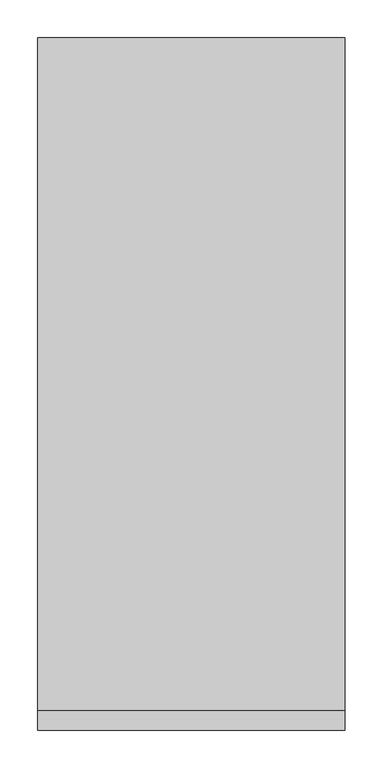
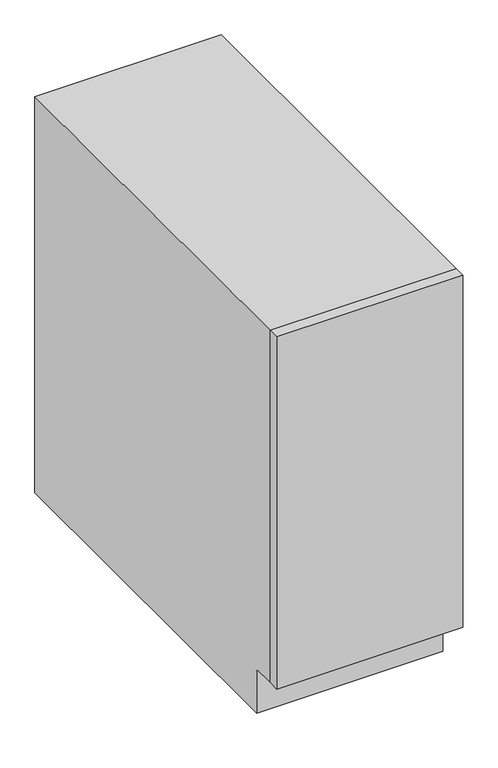
"""IFC4 building model written with IfcOpenShell, lengths in millimetres: furniture geometry, OD_CW_Base Cabinet : OD_CW_Base Cabinet."""

from ifc_helpers import new_model, si_unit, frame, origin, place, context, project, spatial, polyline, outline, extrude, source, transform, mapped, element, save


def furniture_13f5d7f9(model_context):
    return source(origin(), model_context, "Body", "SweptSolid", [
        extrude(outline(polyline([(18.7377049, -279.4), (425.1377049, -279.4), (425.1377049, -304.8), (18.7377049, -304.8), (18.7377049, -279.4)])), frame((0.0, 0.0, 101.6), z_axis=(0.0, 0.0, 1.0), x_axis=(1.0, 0.0, 0.0)), (0.0, 0.0, 1.0), 812.8),
        extrude(outline(polyline([(-279.4, 914.4), (609.6, 914.4), (609.6, 0.0), (-228.6, 0.0), (-228.6, 101.6), (-279.4, 101.6), (-279.4, 914.4)])), frame((18.7377049, 0.0, 0.0), z_axis=(1.0, 0.0, 0.0), x_axis=(0.0, 1.0, 0.0)), (0.0, 0.0, 1.0), 406.4),
    ])


if __name__ == "__main__":
    model = new_model("IFC4")
    model_context = context("Model", 3, world=origin())
    ifc_project = project(units=[si_unit("LENGTHUNIT", "METRE", prefix="MILLI")], contexts=[model_context])
    site = spatial("IfcSite", under=ifc_project)
    building = spatial("IfcBuilding", under=site)
    placement = place(None, origin())
    furniture_shape = furniture_13f5d7f9(model_context)
    element("IfcFurniture", 1, ObjectType="OD_CW_Base Cabinet : OD_CW_Base Cabinet", at=placement, inside=building, context=model_context, shape_type="MappedRepresentation", body=[
        mapped(furniture_shape, transform((0.0, 0.0, 0.0), x_axis=(1.0, 0.0, 0.0), y_axis=(0.0, 1.0, 0.0), z_axis=(0.0, 0.0, 1.0))),
    ])
    save(model, "model.ifc")

# Revit data of these elements
# Type "OD_CW_Base Cabinet : OD_CW_Base Cabinet"
#   OD_CW_Width [instance default] = 2' - 10"
#   OD_CW_Length [instance default] = 8' - 0"
#   OD_CW_Height [instance default] = 2' - 3"
#   Depth = 2' - 0"
#   Height = 3' - 0"
#   Width = 4' - 0"
#   OD_CW_Material_Front Panel [instance default] = none
#   OD_CW_Material_Body [instance default] = none
# Element 1 (IfcFurniture, "OD_CW_Base Cabinet : OD_CW_Base Cabinet")
#   OD_CW_Width = 3' - 0"
#   OD_CW_Length = 1' - 4"
#   OD_CW_Height = 3' - 0"
#   OD_CW_Material_Body = FRYER
#   Materials on its faces: "FRYER", "CASEWORK"
# Materials
#   "FRYER": class "Generic", colour RGB 187 187 187, transparency 0, Cost = 0
#   "CASEWORK": class "Generic", colour RGB 181 181 181, transparency 0, Cost = 0
